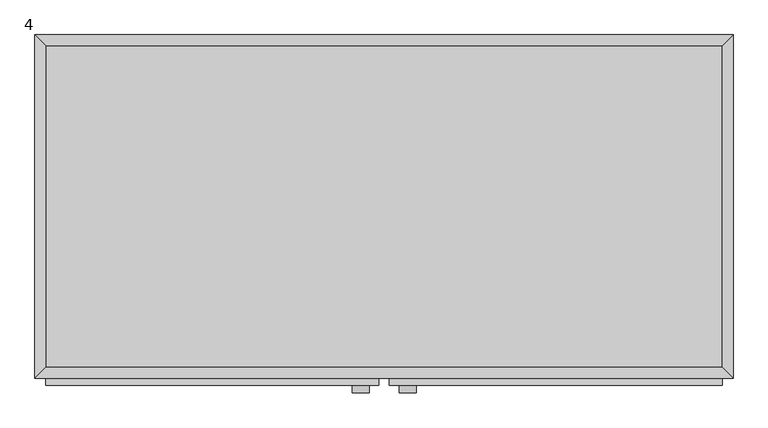
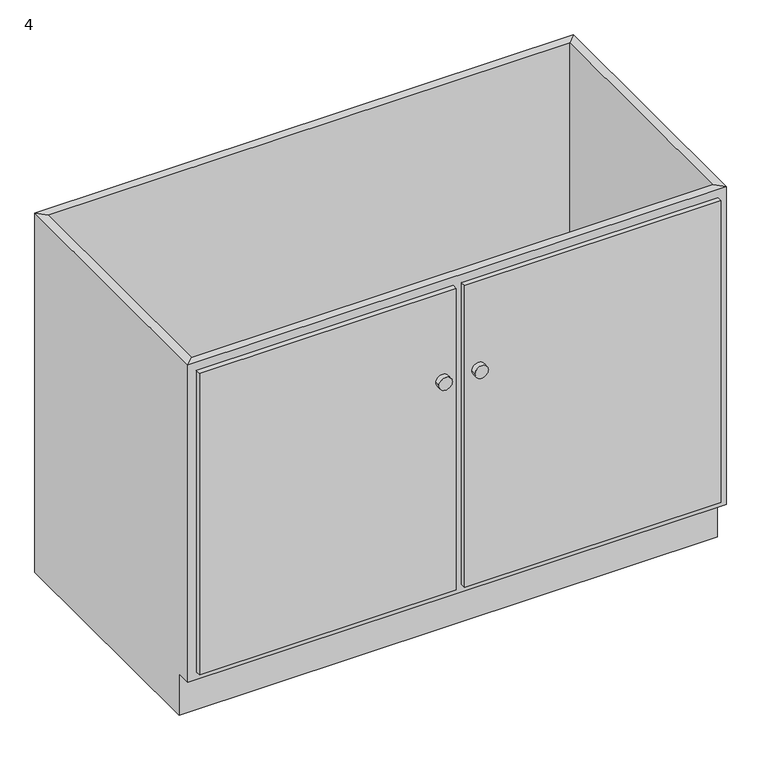
"""IFC4 building model written with IfcOpenShell, lengths in millimetres: furniture geometry, M_Base Cabinet-Double Door & 2 Drawer-round : 4."""

from ifc_helpers import new_model, si_unit, point, frame, frame_2d, origin, place, context, project, spatial, polyline, circle_curve, trimmed, segment, composite_curve, outline, extrude, faceted_brep, source, transform, mapped, element, save


def furniture_4_095f2b8e(model_context):
    return source(origin(), model_context, "Body", "SolidModel", [
        faceted_brep([(609.2877049, -580.95, 860.0), (609.2877049, -580.95, 100.0), (-571.8122951, -580.95, 100.0), (-571.8122951, -580.95, 860.0), (-590.8622951, -600.0, 860.0), (628.3377049, -600.0, 860.0), (-590.8622951, -600.0, 100.0), (628.3377049, -600.0, 100.0), (-571.8122951, -565.0, 100.0), (-571.8122951, -19.05, 100.0), (-571.8122951, -19.05, 860.0), (-590.8622951, 0.0, 860.0), (-590.8622951, 0.0, 0.0), (-590.8622951, -565.0, 0.0), (-590.8622951, -565.0, 100.0), (609.2877049, -19.05, 100.0), (609.2877049, -19.05, 860.0), (628.3377049, 0.0, 860.0), (628.3377049, 0.0, 0.0), (609.2877049, -565.0, 100.0), (628.3377049, -565.0, 100.0), (628.3377049, -565.0, 0.0)], [[[0, 1, 2, 3]], [[0, 3, 4, 5]], [[5, 4, 6, 7]], [[2, 1, 7, 6]], [[3, 2, 8, 9, 10]], [[4, 3, 10, 11]], [[6, 4, 11, 12, 13, 14]], [[2, 6, 14, 8]], [[10, 9, 15, 16]], [[11, 10, 16, 17]], [[12, 11, 17, 18]], [[1, 0, 16, 15, 19]], [[0, 5, 17, 16]], [[5, 7, 20, 21, 18, 17]], [[7, 1, 19, 20]], [[8, 19, 15, 9]], [[18, 21, 13, 12]], [[13, 21, 20, 19, 8, 14]]]),
        extrude(outline(composite_curve([segment(trimmed(circle_curve(frame_2d((631.4, 60.0127049)), 15.0), [point((631.4, 45.0127049))], [point((631.4, 75.0127049))], False, "CARTESIAN"), True, "CONTINUOUS"), segment(trimmed(circle_curve(frame_2d((631.4, 60.0127049)), 15.0), [point((631.4, 75.0127049))], [point((631.4, 45.0127049))], False, "CARTESIAN"), True, "CONTINUOUS")], self_intersect=False)), frame((0.0, -625.4, 0.0), z_axis=(0.0, 1.0, 0.0), x_axis=(0.0, 0.0, 1.0)), (0.0, 0.0, 1.0), 12.7),
        extrude(outline(composite_curve([segment(trimmed(circle_curve(frame_2d((631.4, -21.5872951)), 15.0), [point((631.4, -36.5872951))], [point((631.4, -6.5872951))], False, "CARTESIAN"), True, "CONTINUOUS"), segment(trimmed(circle_curve(frame_2d((631.4, -21.5872951)), 15.0), [point((631.4, -6.5872951))], [point((631.4, -36.5872951))], False, "CARTESIAN"), True, "CONTINUOUS")], self_intersect=False)), frame((0.0, -625.4, 0.0), z_axis=(0.0, 1.0, 0.0), x_axis=(0.0, 0.0, 1.0)), (0.0, 0.0, 1.0), 12.7),
        extrude(outline(polyline([(9.2127049, -612.7), (-571.8122951, -612.7), (-571.8122951, -600.0), (9.2127049, -600.0), (9.2127049, -612.7)])), frame((0.0, 0.0, 119.05), z_axis=(0.0, 0.0, 1.0), x_axis=(1.0, 0.0, 0.0)), (0.0, 0.0, 1.0), 721.9),
        extrude(outline(polyline([(609.2877049, -612.7), (28.2627049, -612.7), (28.2627049, -600.0), (609.2877049, -600.0), (609.2877049, -612.7)])), frame((0.0, 0.0, 119.05), z_axis=(0.0, 0.0, 1.0), x_axis=(1.0, 0.0, 0.0)), (0.0, 0.0, 1.0), 721.9),
        extrude(outline(polyline([(609.2877049, -19.05), (609.2877049, -580.95), (-571.8122951, -580.95), (-571.8122951, -19.05), (609.2877049, -19.05)])), frame((0.0, 0.0, 100.0), z_axis=(0.0, 0.0, 1.0), x_axis=(1.0, 0.0, 0.0)), (0.0, 0.0, 1.0), 19.05),
    ])


if __name__ == "__main__":
    model = new_model("IFC4")
    model_context = context("Model", 3, world=origin())
    ifc_project = project(units=[si_unit("LENGTHUNIT", "METRE", prefix="MILLI")], contexts=[model_context])
    site = spatial("IfcSite", under=ifc_project)
    building = spatial("IfcBuilding", under=site)
    placement = place(None, origin())
    furniture_4_shape = furniture_4_095f2b8e(model_context)
    element("IfcFurniture", 1, ObjectType="M_Base Cabinet-Double Door & 2 Drawer-round : 4", at=placement, inside=building, context=model_context, shape_type="MappedRepresentation", body=[
        mapped(furniture_4_shape, transform((0.0, 0.0, 0.0), x_axis=(1.0, 0.0, 0.0), y_axis=(0.0, 1.0, 0.0), z_axis=(0.0, 0.0, 1.0))),
    ])
    save(model, "model.ifc")

# Revit data of these elements
# Type "M_Base Cabinet-Double Door & 2 Drawer-round : 4"
#   Depth = 1' - 11.62205"
#   Height = 2' - 9.85827"
#   Plinth Depth = 0' - 1.37795"
#   Plinth Height = 0' - 3.93701"
#   Width = 4' - 0"
#   Cabinet Material = Base cabinet 2120100 Aspekt - 83012120100 - White
#   Door/Drawer Material = Base cabinet 2120100 Aspekt - 83012120100 - White
#   Handle Material = Cabinets - Handles
#   Default Elevation = 0
# Element 1 (IfcFurniture, "M_Base Cabinet-Double Door & 2 Drawer-round : 4")
#   Materials on its faces: "Base cabinet 2120100 Aspekt - 83012120100 - White", "Cabinets - Handles"
# Materials
#   "Base cabinet 2120100 Aspekt - 83012120100 - White": class "Miscellaneous", colour RGB 255 255 255, transparency 0, Manufacturer = "Marbodal", URL = "http://www.marbodal.se", Cost = 0
#   "Cabinets - Handles": class "Metal", colour RGB 57 57 57, transparency 0
